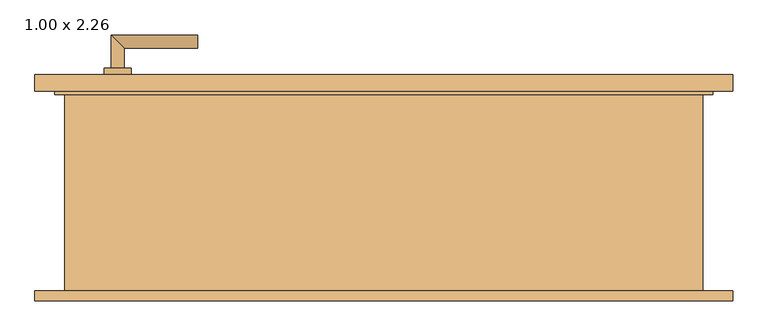
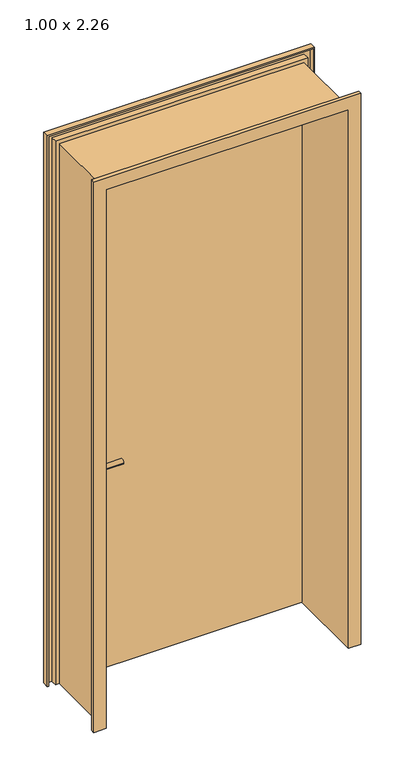
"""IFC4 building model written with IfcOpenShell, lengths in millimetres: door geometry, Drehflügel 1-flg - Stahlzarge : 1.00 x 2.26."""

from ifc_helpers import new_model, si_unit, point, frame, frame_2d, origin, place, context, project, spatial, polyline, circle_curve, ellipse_curve, trimmed, segment, composite_curve, outline, extrude, faceted_brep, source, transform, mapped, element, save
from ifc_brep_helpers import plane_surface, cylinder_surface, advanced_brep


def door_1_00_x_2_26_83e26606(model_context):
    return source(origin(), model_context, "Body", "SolidModel", [
        advanced_brep(
        [(-410.0, 139.4346141, 1000.0), (-390.0, 139.4346141, 1000.0), (-410.0, 69.4346141, 1000.0), (-390.0, 89.4346141, 1000.0), (-280.0, 69.4346141, 1000.0), (-280.0, 89.4346141, 1000.0)],
        [
            (0, 1, circle_curve(frame((-400.0, 139.4346141, 1000.0), z_axis=(0.0, 1.0, 0.0), x_axis=(1.0, 0.0, 0.0)), 10.0)),
            (1, 0, circle_curve(frame((-400.0, 139.4346141, 1000.0), z_axis=(0.0, 1.0, 0.0), x_axis=(1.0, 0.0, 0.0)), 10.0)),
            (0, 2),
            (2, 3, ellipse_curve(frame((-400.0, 79.4346141, 1000.0), z_axis=(-0.7071067811865385, 0.7071067811865565, 0.0), x_axis=(0.7071067811865563, 0.7071067811865386, 0.0)), 14.1421356, 10.0)),
            (3, 1),
            (3, 2, ellipse_curve(frame((-400.0, 79.4346141, 1000.0), z_axis=(-0.7071067811865385, 0.7071067811865565, 0.0), x_axis=(0.7071067811865563, 0.7071067811865386, 0.0)), 14.1421356, 10.0)),
            (4, 5, circle_curve(frame((-280.0, 79.4346141, 1000.0), z_axis=(1.0, 0.0, 0.0), x_axis=(0.0, 1.0, 0.0)), 10.0)),
            (5, 4, circle_curve(frame((-280.0, 79.4346141, 1000.0), z_axis=(1.0, 0.0, 0.0), x_axis=(0.0, 1.0, 0.0)), 10.0)),
            (2, 4),
            (5, 3),
        ],
        [
            plane_surface(frame((-400.0, 139.4346141, -287.7526403), z_axis=(0.0, 1.0, 0.0), x_axis=(0.0, 0.0, 1.0))),
            cylinder_surface(frame((-400.0, 139.4346141, 1000.0), z_axis=(0.0, 1.0, 0.0), x_axis=(1.0, 0.0, 0.0)), 10.0),
            plane_surface(frame((-280.0, 79.4346141, -287.7526403), z_axis=(1.0, 0.0, 0.0), x_axis=(0.0, 0.0, 1.0))),
            cylinder_surface(frame((-400.0, 79.4346141, 1000.0), z_axis=(-1.0, 0.0, 0.0), x_axis=(0.0, 1.0, 0.0)), 10.0),
        ],
        [
            (0, [[1, 2]]),
            (1, [[-1, 3, 4, 5]]),
            (1, [[-2, -5, 6, -3]]),
            (2, [[7, 8]]),
            (3, [[-4, 9, -8, 10]]),
            (3, [[-6, -10, -7, -9]]),
        ],
    ),
        advanced_brep(
        [(-390.0, 199.4346141, 1000.0), (-410.0, 199.4346141, 1000.0), (-390.0, 229.4346141, 1000.0), (-410.0, 249.4346141, 1000.0), (-280.0, 229.4346141, 1000.0), (-280.0, 249.4346141, 1000.0)],
        [
            (0, 1, circle_curve(frame((-400.0, 199.4346141, 1000.0), z_axis=(0.0, -1.0, 0.0), x_axis=(-1.0, 0.0, 0.0)), 10.0)),
            (1, 0, circle_curve(frame((-400.0, 199.4346141, 1000.0), z_axis=(0.0, -1.0, 0.0), x_axis=(-1.0, 0.0, 0.0)), 10.0)),
            (0, 2),
            (2, 3, ellipse_curve(frame((-400.0, 239.4346141, 1000.0), z_axis=(-0.7071067811865475, -0.7071067811865475, 0.0), x_axis=(0.7071067811865474, -0.7071067811865476, 0.0)), 14.1421356, 10.0)),
            (3, 1),
            (3, 2, ellipse_curve(frame((-400.0, 239.4346141, 1000.0), z_axis=(-0.7071067811865475, -0.7071067811865475, 0.0), x_axis=(0.7071067811865474, -0.7071067811865476, 0.0)), 14.1421356, 10.0)),
            (4, 5, circle_curve(frame((-280.0, 239.4346141, 1000.0), z_axis=(1.0, 0.0, 0.0), x_axis=(0.0, 1.0, 0.0)), 10.0)),
            (5, 4, circle_curve(frame((-280.0, 239.4346141, 1000.0), z_axis=(1.0, 0.0, 0.0), x_axis=(0.0, 1.0, 0.0)), 10.0)),
            (2, 4),
            (5, 3),
        ],
        [
            plane_surface(frame((-400.0, 199.4346141, -287.7526403), z_axis=(0.0, -1.0, 0.0), x_axis=(0.0, 0.0, 1.0))),
            cylinder_surface(frame((-400.0, 199.4346141, 1000.0), z_axis=(0.0, -1.0, 0.0), x_axis=(-1.0, 0.0, 0.0)), 10.0),
            plane_surface(frame((-280.0, 239.4346141, -287.7526403), z_axis=(1.0, 0.0, 0.0), x_axis=(0.0, 0.0, 1.0))),
            cylinder_surface(frame((-400.0, 239.4346141, 1000.0), z_axis=(-1.0, 0.0, 0.0), x_axis=(0.0, 1.0, 0.0)), 10.0),
        ],
        [
            (0, [[1, 2]]),
            (1, [[-1, 3, 4, 5]]),
            (1, [[-2, -5, 6, -3]]),
            (2, [[7, 8]]),
            (3, [[-4, 9, -8, 10]]),
            (3, [[-6, -10, -7, -9]]),
        ],
    ),
        extrude(outline(composite_curve([segment(trimmed(circle_curve(frame_2d((1000.0, -400.0)), 20.0), [point((1000.0, -420.0))], [point((1000.0, -380.0))], False, "CARTESIAN"), True, "CONTINUOUS"), segment(trimmed(circle_curve(frame_2d((1000.0, -400.0)), 20.0), [point((1000.0, -380.0))], [point((1000.0, -420.0))], False, "CARTESIAN"), True, "CONTINUOUS")], self_intersect=False)), frame((0.0, 129.4346141, 0.0), z_axis=(0.0, 1.0, 0.0), x_axis=(0.0, 0.0, 1.0)), (0.0, 0.0, 1.0), 10.0),
        extrude(outline(composite_curve([segment(trimmed(circle_curve(frame_2d((1000.0, -400.0)), 20.0), [point((1000.0, -420.0))], [point((1000.0, -380.0))], False, "CARTESIAN"), True, "CONTINUOUS"), segment(trimmed(circle_curve(frame_2d((1000.0, -400.0)), 20.0), [point((1000.0, -380.0))], [point((1000.0, -420.0))], False, "CARTESIAN"), True, "CONTINUOUS")], self_intersect=False)), frame((0.0, 189.4346141, 0.0), z_axis=(0.0, 1.0, 0.0), x_axis=(0.0, 0.0, 1.0)), (0.0, 0.0, 1.0), 10.0),
        extrude(outline(polyline([(490.0, 164.4346141), (-490.0, 164.4346141), (-490.0, 189.4346141), (490.0, 189.4346141), (490.0, 164.4346141)])), frame((0.0, 0.0, 100.0), z_axis=(0.0, 0.0, 1.0), x_axis=(1.0, 0.0, 0.0)), (0.0, 0.0, 1.0), 2250.0),
        faceted_brep([(524.4603207, -150.5653859, 100.0), (475.0, -150.5653859, 100.0), (475.0, 164.4346141, 100.0), (490.0, 164.4346141, 100.0), (490.0, 189.4346141, 100.0), (524.4603207, 189.4346141, 100.0), (524.4603207, 164.4346141, 100.0), (519.4603207, 164.4346141, 100.0), (519.4603207, 184.4346141, 100.0), (495.0, 184.4346141, 100.0), (495.0, 159.4346141, 100.0), (480.0, 159.4346141, 100.0), (480.0, -145.5653859, 100.0), (519.4603207, -145.5653859, 100.0), (519.4603207, -135.5653859, 100.0), (524.4603207, -135.5653859, 100.0), (524.4603207, -150.5653859, 2384.4603207), (-524.4603207, -150.5653859, 2384.4603207), (-524.4603207, -150.5653859, 100.0), (-475.0, -150.5653859, 100.0), (-475.0, -150.5653859, 2335.0), (475.0, -150.5653859, 2335.0), (475.0, 164.4346141, 2335.0), (-475.0, 164.4346141, 2335.0), (-475.0, 164.4346141, 100.0), (-490.0, 164.4346141, 100.0), (-490.0, 164.4346141, 2350.0), (490.0, 164.4346141, 2350.0), (490.0, 189.4346141, 2350.0), (-490.0, 189.4346141, 2350.0), (-490.0, 189.4346141, 100.0), (-524.4603207, 189.4346141, 100.0), (-524.4603207, 189.4346141, 2384.4603207), (524.4603207, 189.4346141, 2384.4603207), (524.4603207, 164.4346141, 2384.4603207), (-524.4603207, 164.4346141, 2384.4603207), (-524.4603207, 164.4346141, 100.0), (-519.4603207, 164.4346141, 100.0), (-519.4603207, 164.4346141, 2379.4603207), (519.4603207, 164.4346141, 2379.4603207), (519.4603207, 184.4346141, 2379.4603207), (-519.4603207, 184.4346141, 2379.4603207), (-519.4603207, 184.4346141, 100.0), (-495.0, 184.4346141, 100.0), (-495.0, 184.4346141, 2355.0), (495.0, 184.4346141, 2355.0), (495.0, 159.4346141, 2355.0), (-495.0, 159.4346141, 2355.0), (-495.0, 159.4346141, 100.0), (-480.0, 159.4346141, 100.0), (-480.0, 159.4346141, 2340.0), (480.0, 159.4346141, 2340.0), (480.0, -145.5653859, 2340.0), (-480.0, -145.5653859, 2340.0), (-480.0, -145.5653859, 100.0), (-519.4603207, -145.5653859, 100.0), (-519.4603207, -145.5653859, 2379.4603207), (519.4603207, -145.5653859, 2379.4603207), (519.4603207, -135.5653859, 2379.4603207), (-519.4603207, -135.5653859, 2379.4603207), (-519.4603207, -135.5653859, 100.0), (-524.4603207, -135.5653859, 100.0), (-524.4603207, -135.5653859, 2384.4603207), (524.4603207, -135.5653859, 2384.4603207)], [[[0, 1, 2, 3, 4, 5, 6, 7, 8, 9, 10, 11, 12, 13, 14, 15]], [[1, 0, 16, 17, 18, 19, 20, 21]], [[2, 1, 21, 22]], [[3, 2, 22, 23, 24, 25, 26, 27]], [[4, 3, 27, 28]], [[5, 4, 28, 29, 30, 31, 32, 33]], [[6, 5, 33, 34]], [[7, 6, 34, 35, 36, 37, 38, 39]], [[8, 7, 39, 40]], [[9, 8, 40, 41, 42, 43, 44, 45]], [[10, 9, 45, 46]], [[11, 10, 46, 47, 48, 49, 50, 51]], [[12, 11, 51, 52]], [[13, 12, 52, 53, 54, 55, 56, 57]], [[14, 13, 57, 58]], [[15, 14, 58, 59, 60, 61, 62, 63]], [[0, 15, 63, 16]], [[17, 62, 61, 18]], [[18, 61, 60, 55, 54, 49, 48, 43, 42, 37, 36, 31, 30, 25, 24, 19]], [[23, 20, 19, 24]], [[29, 26, 25, 30]], [[35, 32, 31, 36]], [[41, 38, 37, 42]], [[47, 44, 43, 48]], [[53, 50, 49, 54]], [[59, 56, 55, 60]], [[22, 21, 20, 23]], [[28, 27, 26, 29]], [[34, 33, 32, 35]], [[40, 39, 38, 41]], [[46, 45, 44, 47]], [[52, 51, 50, 53]], [[58, 57, 56, 59]], [[16, 63, 62, 17]]]),
    ])


if __name__ == "__main__":
    model = new_model("IFC4")
    model_context = context("Model", 3, world=origin())
    ifc_project = project(units=[si_unit("LENGTHUNIT", "METRE", prefix="MILLI")], contexts=[model_context])
    site = spatial("IfcSite", under=ifc_project)
    building = spatial("IfcBuilding", under=site)
    placement = place(None, origin())
    door_1_00_x_2_26_shape = door_1_00_x_2_26_83e26606(model_context)
    element("IfcDoor", 1, ObjectType="Drehflügel 1-flg - Stahlzarge : 1.00 x 2.26", at=placement, inside=building, context=model_context, shape_type="MappedRepresentation", body=[
        mapped(door_1_00_x_2_26_shape, transform((0.0, 0.0, 0.0), x_axis=(1.0, 0.0, 0.0), y_axis=(0.0, 1.0, 0.0), z_axis=(0.0, 0.0, 1.0))),
    ])
    save(model, "model.ifc")

# Revit data of these elements
# Type "Drehflügel 1-flg - Stahlzarge : 1.00 x 2.26"
#   Construction Type Id = "MDOOR"
#   Type Mark = "20"
#   Operation = "SingleSwingRight"
#   Keynote = "16.03"
#   Analytic Construction = "Metall"
#   Thermal Resistance (R) = 0.270117 (m²·K)/W
#   Heat Transfer Coefficient (U) = 3.7021 W/(m²·K)
#   Rough Width = 1.000 m
#   Rough Height [instance default] = 2.360 m
#   Höhe Türgriff [instance default] = 0.900 m
#   Height = 2.260 m
#   Fußbodenaufbau [instance default] = 0.100 m
#   Width = 1.000 m
#   Sichtbarkeit Sturzlinien [instance default] = yes
#   Türgriff auswählen [instance default] = element 221079
#   Türgriff [instance default] = none
#   Türflügel [instance default] = none
#   Rahmen/Pfosten [instance default] = Metall - Lackiert - Grau
#   Visual Light Transmittance = 0
#   Solar Heat Gain Coefficient = 0
#   Function = (empty or 0)
#   Wall Closure = (empty or 0)
# Element 1 (IfcDoor, "Drehflügel 1-flg - Stahlzarge : 1.00 x 2.26")
#   Materials on its faces: "Metall - Lackiert - Grau", "Metall - Chrom", "Holz - Birke"
# Materials
#   "Metall - Lackiert - Grau": class "Farbe 1", colour RGB 98 98 98, transparency 0, Cost = 0
#   "Metall - Chrom": class "Metall", colour RGB 247 247 247, transparency 0, Cost = 0
#   "Holz - Birke": class "Holz", colour RGB 213 164 103, transparency 0, Cost = 0
